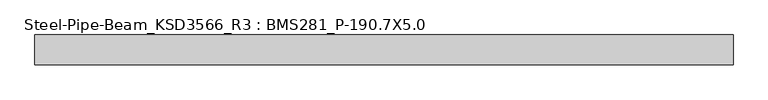
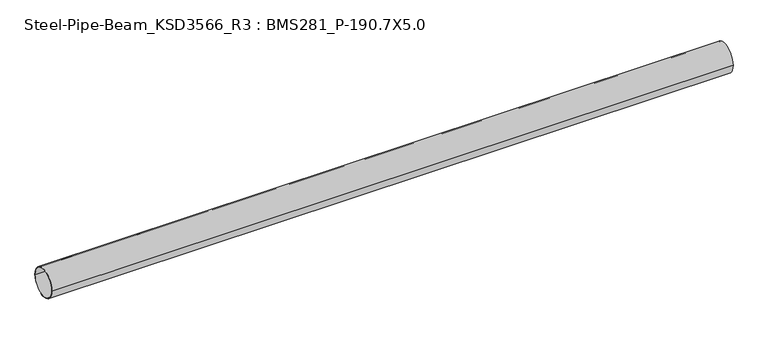
"""IFC4 building model written with IfcOpenShell, lengths in millimetres: member geometry, Steel-Pipe-Beam_KSD3566_R3 : BMS281_P-190.7X5.0."""

from ifc_helpers import new_model, si_unit, point, frame, origin, origin_2d, place, context, project, spatial, circle_curve, trimmed, segment, composite_curve, outline, extrude, source, transform, mapped, element, save


def steel_pipe_beam_ksd3566_r3_bms281_p_190_7x5_0_e7085745(model_context):
    return source(origin(), model_context, "Body", "SweptSolid", [
        extrude(outline(composite_curve([segment(trimmed(circle_curve(origin_2d(), 95.35), [point((-95.35, 0.0))], [point((95.35, 0.0))], False, "CARTESIAN"), True, "CONTINUOUS"), segment(trimmed(circle_curve(origin_2d(), 95.35), [point((95.35, 0.0))], [point((-95.35, 0.0))], False, "CARTESIAN"), True, "CONTINUOUS")], self_intersect=False), holes=[composite_curve([segment(trimmed(circle_curve(origin_2d(), 90.35), [point((90.35, 0.0))], [point((-90.35, 0.0))], True, "CARTESIAN"), True, "CONTINUOUS"), segment(trimmed(circle_curve(origin_2d(), 90.35), [point((-90.35, 0.0))], [point((90.35, 0.0))], True, "CARTESIAN"), True, "CONTINUOUS")], self_intersect=False)]), frame((-2215.2447119, 0.0, 0.0), z_axis=(1.0, 0.0, 0.0), x_axis=(0.0, 1.0, 0.0)), (0.0, 0.0, 1.0), 4448.4931366),
    ])


if __name__ == "__main__":
    model = new_model("IFC4")
    model_context = context("Model", 3, world=origin())
    ifc_project = project(units=[si_unit("LENGTHUNIT", "METRE", prefix="MILLI")], contexts=[model_context])
    site = spatial("IfcSite", under=ifc_project)
    building = spatial("IfcBuilding", under=site)
    placement = place(None, origin())
    steel_pipe_beam_ksd3566_r3_bms281_p_190_7x5_0_shape = steel_pipe_beam_ksd3566_r3_bms281_p_190_7x5_0_e7085745(model_context)
    element("IfcMember", 1, ObjectType="Steel-Pipe-Beam_KSD3566_R3 : BMS281_P-190.7X5.0", at=placement, inside=building, context=model_context, shape_type="MappedRepresentation", body=[
        mapped(steel_pipe_beam_ksd3566_r3_bms281_p_190_7x5_0_shape, transform((0.0, 0.0, 0.0), x_axis=(1.0, 0.0, 0.0), y_axis=(0.0, 1.0, 0.0), z_axis=(0.0, 0.0, 1.0))),
    ])
    save(model, "model.ifc")

# Revit data of these elements
# Type "Steel-Pipe-Beam_KSD3566_R3 : BMS281_P-190.7X5.0"
#   Keynote = "P-190.7X5.0"
#   SteelWeight = "Light"
#   t = 0.0050 m
#   Surface Area = 0.599102 m²/m
#   Section Area = 29.1697 cm²
#   Mass per Unit Length = 22.8982 kg/m
#   Length [instance default] = 1.5000 m
#   D = 0.1907 m
#   hec_material4 [instance default] = none
#   hec_material3 [instance default] = none
#   hec_material2 [instance default] = none
#   hec_material1 [instance default] = none
#   Structural Material [instance default] = Steel, 45-345
#   Assembly Code = ""
# Element 1 (IfcMember, "Steel-Pipe-Beam_KSD3566_R3 : BMS281_P-190.7X5.0")
#   Structural Material = none
# Materials
#   "Steel, 45-345": class "Metal", colour RGB 189 187 185, transparency 0, Description = "Steel 345 MPa", Cost = 0
